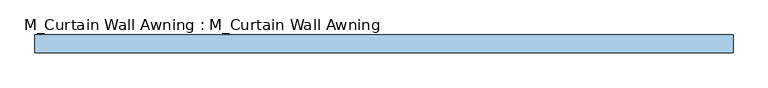
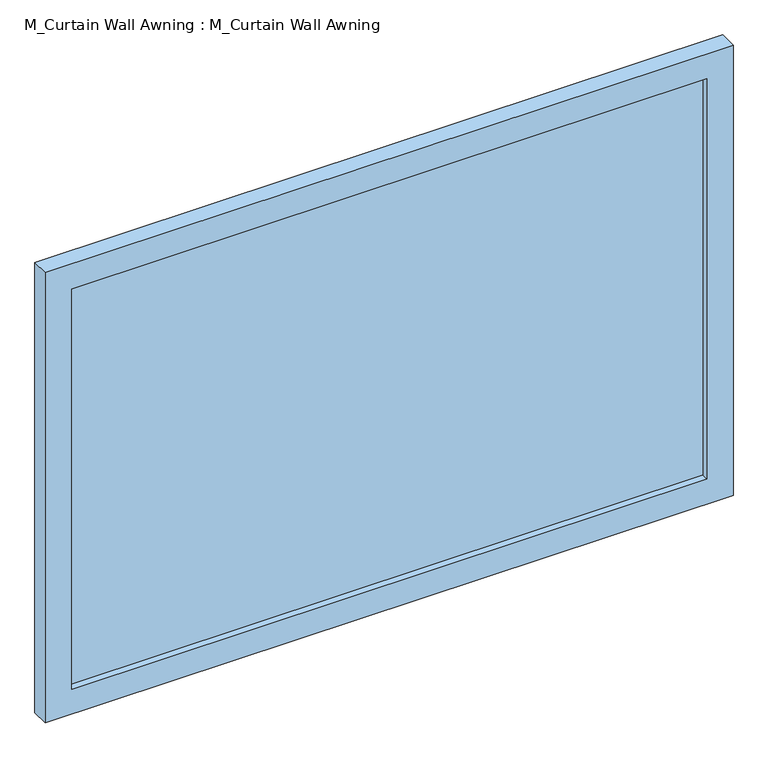
"""IFC4 building model written with IfcOpenShell, lengths in millimetres: window geometry, M_Curtain Wall Awning : M_Curtain Wall Awning."""

from ifc_helpers import new_model, si_unit, frame, origin, place, context, project, spatial, polyline, outline, extrude, source, transform, mapped, element, save


def m_curtain_wall_awning_m_curtain_wall_awning_db665c81(model_context):
    return source(origin(), model_context, "Body", "SweptSolid", [
        extrude(outline(polyline([(900.0, 44.05), (-900.0, 44.05), (-900.0, 56.75), (900.0, 56.75), (900.0, 44.05)])), frame((0.0, 0.0, 75.0), z_axis=(0.0, 0.0, 1.0), x_axis=(1.0, 0.0, 0.0)), (0.0, 0.0, 1.0), 1200.0),
        extrude(outline(polyline([(1350.0, -975.0), (0.0, -975.0), (0.0, 975.0), (1350.0, 975.0), (1350.0, -975.0)]), holes=[polyline([(1275.0, -900.0), (1275.0, 900.0), (75.0, 900.0), (75.0, -900.0), (1275.0, -900.0)])]), frame((0.0, 25.0, 0.0), z_axis=(0.0, 1.0, 0.0), x_axis=(0.0, 0.0, 1.0)), (0.0, 0.0, 1.0), 50.0),
    ])


if __name__ == "__main__":
    model = new_model("IFC4")
    model_context = context("Model", 3, world=origin())
    ifc_project = project(units=[si_unit("LENGTHUNIT", "METRE", prefix="MILLI")], contexts=[model_context])
    site = spatial("IfcSite", under=ifc_project)
    building = spatial("IfcBuilding", under=site)
    placement = place(None, origin())
    m_curtain_wall_awning_m_curtain_wall_awning_shape = m_curtain_wall_awning_m_curtain_wall_awning_db665c81(model_context)
    element("IfcWindow", 1, ObjectType="M_Curtain Wall Awning : M_Curtain Wall Awning", at=placement, inside=building, context=model_context, shape_type="MappedRepresentation", body=[
        mapped(m_curtain_wall_awning_m_curtain_wall_awning_shape, transform((0.0, 0.0, 0.0), x_axis=(1.0, 0.0, 0.0), y_axis=(0.0, 1.0, 0.0), z_axis=(0.0, 0.0, 1.0))),
    ])
    save(model, "model.ifc")

# Revit data of these elements
# Type "M_Curtain Wall Awning : M_Curtain Wall Awning"
#   Type Mark = "20"
#   Offset = 0.075 m
#   Sash Width = 0.075 m
#   Thickness = 0.050 m
#   Define Thermal Properties by = 1
#   Glass Pane Material = Window - Glass
#   Sash Material = Metal - Aluminum
# Element 1 (IfcWindow, "M_Curtain Wall Awning : M_Curtain Wall Awning")
#   Materials on its faces: "Metal - Aluminum", "Window - Glass"
# Materials
#   "Window - Glass": class "Glas", colour RGB 128 128 255, transparency 0.75
#   "Metal - Aluminum": class "Unassigned", colour RGB 247 247 247, transparency 0, Comments = "Rendering appearance not upgraded "
